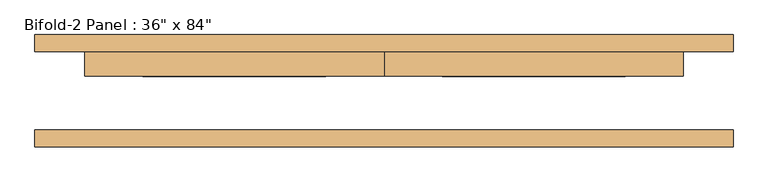
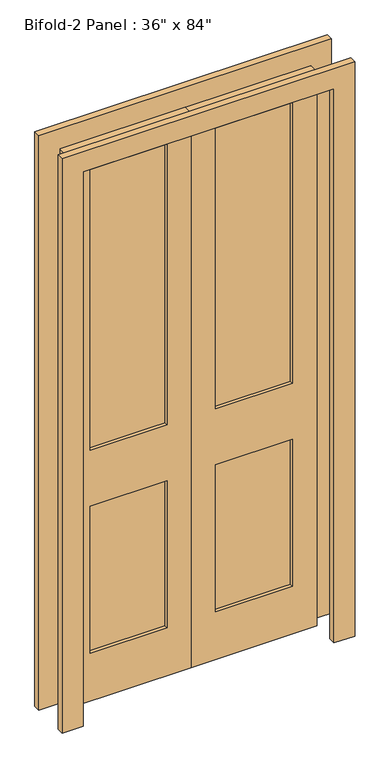
"""IFC4 building model written with IfcOpenShell, lengths in millimetres: door geometry."""

import ifcopenshell
import ifcopenshell.guid

model = None  # the IFC model being written
_history = None  # IfcOwnerHistory: only IFC2X3 demands one
_inside = {}  # id of a spatial element -> (the spatial element, [elements in it])
_under = {}  # id of a project, library or spatial element -> (it, [spatial elements below it])
_declared = {}  # id of a project -> (the project, [libraries it declares])
_typed = {}  # id of a type object -> (the type object, [elements of that type])
_made_of = {}  # id of a material, layer set ... -> (it, [elements and type objects made of it])


def new_model(schema):
    """Start an empty IFC model of exactly this schema.

    Asked for "IFC4X3", IfcOpenShell would pick the latest addendum, in which some entities
    have other attributes; the version numbers below select the first issue.
    IFC2X3 requires an IfcOwnerHistory on every rooted entity: one is made here for all.
    """
    global model, _history
    if schema == "IFC4X3":
        model = ifcopenshell.file(schema_version=(4, 3, 0, 0))
    else:
        model = ifcopenshell.file(schema=schema)
    _inside.clear()
    _under.clear()
    _declared.clear()
    _typed.clear()
    _made_of.clear()
    _history = None
    if model.schema == "IFC2X3":
        org = make("IfcOrganization", Name="unknown")
        user = make(
            "IfcPersonAndOrganization",
            ThePerson=make("IfcPerson", FamilyName="unknown"),
            TheOrganization=org,
        )
        app = make(
            "IfcApplication",
            ApplicationDeveloper=org,
            Version="unknown",
            ApplicationFullName="unknown",
            ApplicationIdentifier="unknown",
        )
        _history = make(
            "IfcOwnerHistory",
            OwningUser=user,
            OwningApplication=app,
            ChangeAction="ADDED",
            CreationDate=0,
        )
    return model


def make(cls, **values):
    """One entity of the class cls with the attributes given. An attribute that is None is left unset."""
    return model.create_entity(
        cls, **{name: value for name, value in values.items() if value is not None}
    )


def rooted(cls, **values):
    """An entity with a GlobalId (a new one), such as an element, a storey or a relation."""
    return make(cls, GlobalId=ifcopenshell.guid.new(), OwnerHistory=_history, **values)


def si_unit(unit_type, name, prefix=None):
    """IfcSIUnit, for example si_unit("LENGTHUNIT", "METRE", prefix="MILLI")."""
    return make("IfcSIUnit", UnitType=unit_type, Prefix=prefix, Name=name)


def assignment(units):
    """IfcUnitAssignment: the units of a project."""
    return None if units is None else make("IfcUnitAssignment", Units=units)


def point(xyz):
    """IfcCartesianPoint."""
    return None if xyz is None else make("IfcCartesianPoint", Coordinates=xyz)


def direction(xyz):
    """IfcDirection."""
    return None if xyz is None else make("IfcDirection", DirectionRatios=xyz)


def frame(location, z_axis=None, x_axis=None):
    """IfcAxis2Placement3D, a coordinate frame: its origin and axes. An axis left out is left unset."""
    return make(
        "IfcAxis2Placement3D",
        Location=point(location),
        Axis=direction(z_axis),
        RefDirection=direction(x_axis),
    )


def origin():
    """The frame at (0, 0, 0) with its axes left unset."""
    return frame((0.0, 0.0, 0.0))


def place(relative_to, where):
    """IfcLocalPlacement: puts the frame where relative to a parent placement (None: the world)."""
    return make(
        "IfcLocalPlacement", PlacementRelTo=relative_to, RelativePlacement=where
    )


def context(
    kind, dimensions, precision=None, world=None, true_north=None, identifier=None
):
    """IfcGeometricRepresentationContext, for example the 3D "Model" context."""
    return make(
        "IfcGeometricRepresentationContext",
        ContextIdentifier=identifier,
        ContextType=kind,
        CoordinateSpaceDimension=dimensions,
        Precision=precision,
        WorldCoordinateSystem=world,
        TrueNorth=true_north,
    )


def project(units=None, contexts=None):
    """IfcProject with its units and contexts."""
    return rooted(
        "IfcProject",
        Name="project",
        RepresentationContexts=contexts,
        UnitsInContext=assignment(units),
    )


def spatial(cls, under=None, at=None, **own):
    """A site, building, storey or space (cls), placed at a placement, below another one or the project."""
    s = rooted(cls, ObjectPlacement=at, **own)
    if under is not None:
        _under.setdefault(under.id(), (under, []))[1].append(s)
    return s


def polyline(points):
    """IfcPolyline through the points."""
    return make("IfcPolyline", Points=[point(p) for p in points])


def outline(outer, holes=None, kind="AREA"):
    """IfcArbitraryClosedProfileDef: a profile drawn as a closed curve; with holes, ...WithVoids."""
    if holes is None:
        return make("IfcArbitraryClosedProfileDef", ProfileType=kind, OuterCurve=outer)
    return make(
        "IfcArbitraryProfileDefWithVoids",
        ProfileType=kind,
        OuterCurve=outer,
        InnerCurves=holes,
    )


def extrude(swept, where, along, depth):
    """IfcExtrudedAreaSolid: the profile swept, set in the frame where, extruded along a direction by depth."""
    return make(
        "IfcExtrudedAreaSolid",
        SweptArea=swept,
        Position=where,
        ExtrudedDirection=direction(along),
        Depth=depth,
    )


def shape(context_of_items, identifier, shape_type, items):
    """IfcShapeRepresentation: the items that make up one representation, for example the "Body"."""
    return make(
        "IfcShapeRepresentation",
        ContextOfItems=context_of_items,
        RepresentationIdentifier=identifier,
        RepresentationType=shape_type,
        Items=items,
    )


def source(mapping_origin, context_of_items, identifier, shape_type, items):
    """IfcRepresentationMap: a shape defined once, which mapped items show again and again."""
    return make(
        "IfcRepresentationMap",
        MappingOrigin=mapping_origin,
        MappedRepresentation=shape(context_of_items, identifier, shape_type, items),
    )


def transform(
    local_origin,
    x_axis=None,
    y_axis=None,
    z_axis=None,
    scale=None,
    scale2=None,
    scale3=None,
    uniform=True,
):
    """IfcCartesianTransformationOperator3D, or its non-uniform kind. x_axis, y_axis, z_axis: its Axis1, 2, 3."""
    if uniform:
        return make(
            "IfcCartesianTransformationOperator3D",
            Axis1=direction(x_axis),
            Axis2=direction(y_axis),
            LocalOrigin=point(local_origin),
            Scale=scale,
            Axis3=direction(z_axis),
        )
    return make(
        "IfcCartesianTransformationOperator3DnonUniform",
        Axis1=direction(x_axis),
        Axis2=direction(y_axis),
        LocalOrigin=point(local_origin),
        Scale=scale,
        Axis3=direction(z_axis),
        Scale2=scale2,
        Scale3=scale3,
    )


def mapped(mapping_source, mapping_target):
    """IfcMappedItem: shows the shape of a source again, moved by a transform."""
    return make(
        "IfcMappedItem", MappingSource=mapping_source, MappingTarget=mapping_target
    )


def made_of(thing, what):
    """Note that an element or type object is made of a material, layer set ...; save() writes the relation."""
    if what is not None:
        _made_of.setdefault(what.id(), (what, []))[1].append(thing)
    return thing


def element(
    cls,
    number,
    at=None,
    inside=None,
    cuts=None,
    type_object=None,
    material=None,
    context=None,
    identifier="Body",
    shape_type=None,
    held_by="IfcProductDefinitionShape",
    body=None,
    shapes=None,
    **own,
):
    """One element of the class cls, such as IfcWall. Its Tag is "e" and its number.

    at: its placement. inside: the storey or other place that contains it. cuts: it is an
    opening in that element (IfcRelVoidsElement). A single representation is given by context,
    identifier, shape_type and body (its items); several are given by shapes. held_by: the class
    of the entity that holds the representations. save() writes the other relations.
    """
    e = rooted(cls, Tag="e%d" % number, ObjectPlacement=at, **own)
    if body is not None:
        shapes = [shape(context, identifier, shape_type, body)]
    if shapes is not None:
        e.Representation = make(held_by, Representations=shapes)
    if inside is not None:
        _inside.setdefault(inside.id(), (inside, []))[1].append(e)
    if cuts is not None:
        rooted(
            "IfcRelVoidsElement", RelatingBuildingElement=cuts, RelatedOpeningElement=e
        )
    if type_object is not None:
        _typed.setdefault(type_object.id(), (type_object, []))[1].append(e)
    return made_of(e, material)


def aggregate(whole, parts):
    """IfcRelAggregates: a whole, such as a stair, and the parts it consists of."""
    return rooted("IfcRelAggregates", RelatingObject=whole, RelatedObjects=parts)


def save(model, path):
    """Write the relations noted so far, then the file.

    IfcRelAggregates (storeys below a building ...), IfcRelContainedInSpatialStructure (elements
    in a storey), IfcRelDefinesByType, IfcRelAssociatesMaterial and IfcRelDeclares: one each for
    every whole, place, type object, material and project.
    """
    for whole, parts in _under.values():
        aggregate(whole, parts)
    for where, things in _inside.values():
        rooted(
            "IfcRelContainedInSpatialStructure",
            RelatedElements=things,
            RelatingStructure=where,
        )
    for kind, things in _typed.values():
        rooted("IfcRelDefinesByType", RelatedObjects=things, RelatingType=kind)
    for what, things in _made_of.values():
        rooted("IfcRelAssociatesMaterial", RelatedObjects=things, RelatingMaterial=what)
    for by, libraries in _declared.values():
        rooted("IfcRelDeclares", RelatingContext=by, RelatedDefinitions=libraries)
    model.write(path)


def door_80e19791(model_context):
    return source(origin(), model_context, "Body", "SweptSolid", [
        extrude(outline(polyline([(2133.6, 0.0), (2133.6, -457.2), (0.0, -457.2), (0.0, 0.0), (2133.6, 0.0)]), holes=[polyline([(2044.7, -88.9), (965.11872, -88.9), (965.11872, -368.3), (2044.7, -368.3), (2044.7, -88.9)]), polyline([(749.3, -88.9), (184.15, -88.9), (184.15, -368.3), (749.3, -368.3), (749.3, -88.9)])]), frame((0.0, 22.225, 0.0), z_axis=(0.0, 1.0, 0.0), x_axis=(0.0, 0.0, 1.0)), (0.0, 0.0, 1.0), 38.1),
        extrude(outline(polyline([(-88.9, 34.925), (-368.3, 34.925), (-368.3, 47.625), (-88.9, 47.625), (-88.9, 34.925)])), frame((0.0, 0.0, 965.11872), z_axis=(0.0, 0.0, 1.0), x_axis=(1.0, 0.0, 0.0)), (0.0, 0.0, 1.0), 1079.58128),
        extrude(outline(polyline([(-88.9, 34.925), (-368.3, 34.925), (-368.3, 47.625), (-88.9, 47.625), (-88.9, 34.925)])), frame((0.0, 0.0, 184.15), z_axis=(0.0, 0.0, 1.0), x_axis=(1.0, 0.0, 0.0)), (0.0, 0.0, 1.0), 565.15),
        extrude(outline(polyline([(368.3, 34.925), (88.9, 34.925), (88.9, 47.625), (368.3, 47.625), (368.3, 34.925)])), frame((0.0, 0.0, 965.11872), z_axis=(0.0, 0.0, 1.0), x_axis=(1.0, 0.0, 0.0)), (0.0, 0.0, 1.0), 1079.58128),
        extrude(outline(polyline([(368.3, 34.925), (88.9, 34.925), (88.9, 47.625), (368.3, 47.625), (368.3, 34.925)])), frame((0.0, 0.0, 184.15), z_axis=(0.0, 0.0, 1.0), x_axis=(1.0, 0.0, 0.0)), (0.0, 0.0, 1.0), 565.15),
        extrude(outline(polyline([(2209.8, -533.4), (0.0, -533.4), (0.0, -457.2), (2133.6, -457.2), (2133.6, 457.2), (0.0, 457.2), (0.0, 533.4), (2209.8, 533.4), (2209.8, -533.4)])), frame((0.0, 60.325, 0.0), z_axis=(0.0, 1.0, 0.0), x_axis=(0.0, 0.0, 1.0)), (0.0, 0.0, 1.0), 25.4),
        extrude(outline(polyline([(2209.8, 533.4), (2209.8, -533.4), (0.0, -533.4), (0.0, -457.2), (2133.6, -457.2), (2133.6, 457.2), (0.0, 457.2), (0.0, 533.4), (2209.8, 533.4)])), frame((0.0, -85.725, 0.0), z_axis=(0.0, 1.0, 0.0), x_axis=(0.0, 0.0, 1.0)), (0.0, 0.0, 1.0), 25.4),
        extrude(outline(polyline([(2133.6, 457.2), (2133.6, 0.0), (0.0, 0.0), (0.0, 457.2), (2133.6, 457.2)]), holes=[polyline([(2044.7, 88.9), (2044.7, 368.3), (965.11872, 368.3), (965.11872, 88.9), (2044.7, 88.9)]), polyline([(749.3, 88.9), (749.3, 368.3), (184.15, 368.3), (184.15, 88.9), (749.3, 88.9)])]), frame((0.0, 22.225, 0.0), z_axis=(0.0, 1.0, 0.0), x_axis=(0.0, 0.0, 1.0)), (0.0, 0.0, 1.0), 38.1),
    ])


if __name__ == "__main__":
    model = new_model("IFC4")
    model_context = context("Model", 3, world=origin())
    ifc_project = project(units=[si_unit("LENGTHUNIT", "METRE", prefix="MILLI")], contexts=[model_context])
    site = spatial("IfcSite", under=ifc_project)
    building = spatial("IfcBuilding", under=site)
    placement = place(None, origin())
    door_shape = door_80e19791(model_context)
    element("IfcDoor", 1, ObjectType="Bifold-2 Panel : 36\" x 84\"", at=placement, inside=building, context=model_context, shape_type="MappedRepresentation", body=[
        mapped(door_shape, transform((0.0, 0.0, 0.0), x_axis=(1.0, 0.0, 0.0), y_axis=(0.0, 1.0, 0.0), z_axis=(0.0, 0.0, 1.0))),
    ])
    save(model, "model.ifc")

# Revit data of these elements
# Type "Bifold-2 Panel : 36\" x 84\""
#   Type Mark = "8"
#   Construction Type Id = "MDOOR"
#   Assembly Code = "C1020"
#   Analytic Construction = "Metal"
#   Thickness = 0' - 1 1/2"
#   Thermal Resistance (R) = 1.5338 (h·ft²·°F)/BTU
#   Heat Transfer Coefficient (U) = 0.651978 BTU/(h·ft²·°F)
#   Height = 7' - 0"
#   Trim Projection Ext = 0' - 1"
#   Trim Projection Int = 0' - 1"
#   Trim Width = 0' - 3"
#   Width = 3' - 0"
#   Define Thermal Properties by = 1
#   Door Material = Door - Panel
#   Frame Material = Door - Frame
#   Visual Light Transmittance = 0
#   Solar Heat Gain Coefficient = 0
#   Function = (empty or 0)
#   Wall Closure = (empty or 0)
# Element 1 (IfcDoor, "Bifold-2 Panel : 36\" x 84\"")
#   Materials on its faces: "Door - Panel", "Door - Frame"
# Materials
#   "Door - Panel": class "Wood", colour RGB 210 159 95, transparency 0, Cost = 0
#   "Door - Frame": class "Miscellaneous", colour RGB 118 70 51, transparency 0, Cost = 0
